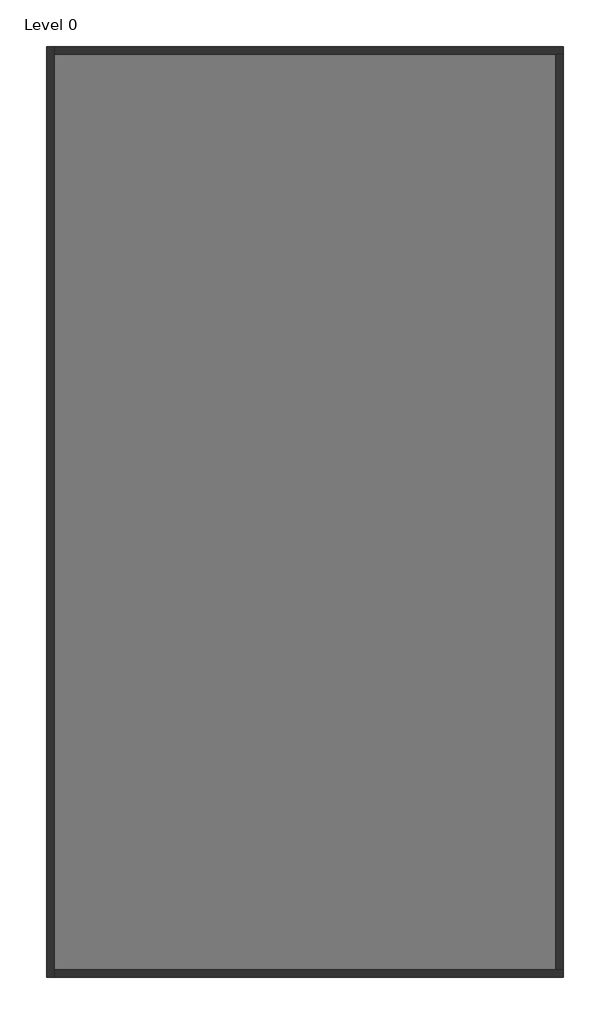
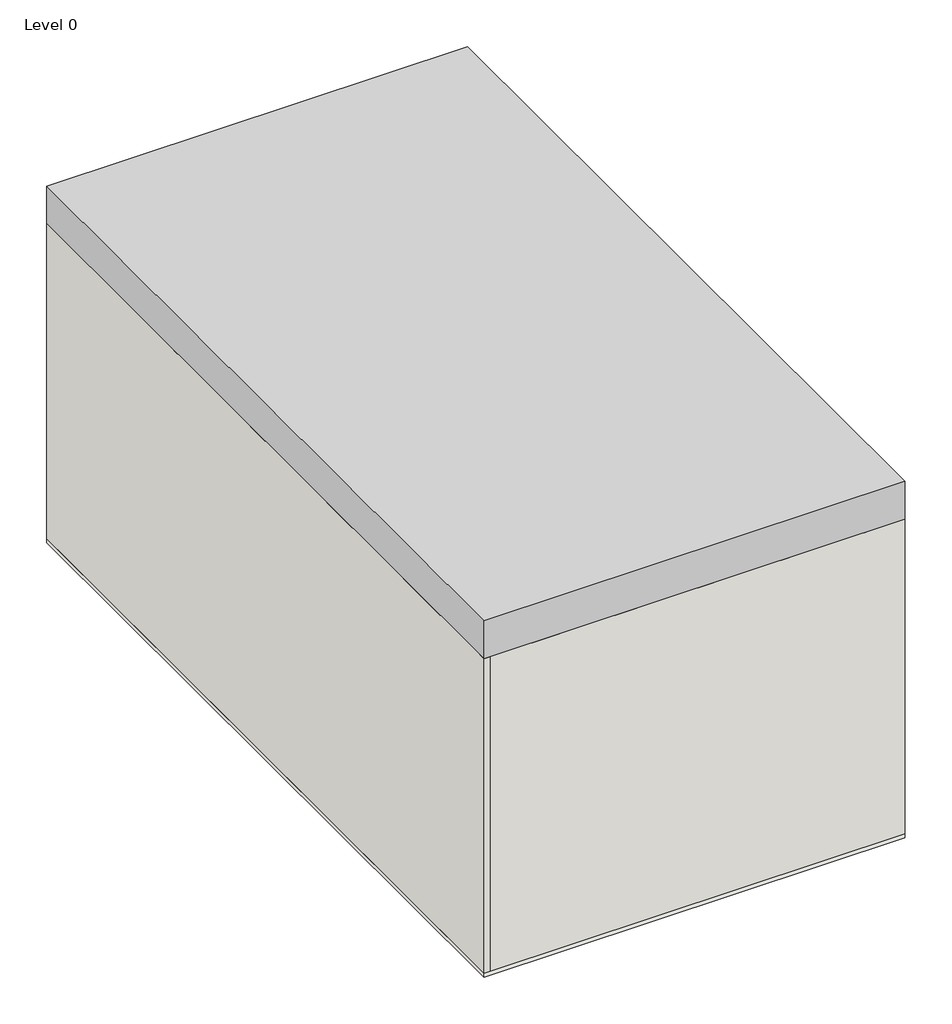
# One storey: 4 walls, 1 proxy, 1 slab.
"""IFC4 building model written with IfcOpenShell, lengths in millimetres."""

from ifc_helpers import new_model, si_unit, frame, origin, origin_with_axes, place, context, project, spatial, polyline, outline, extrude, faceted_brep, element, save

model = new_model("IFC4")

# Units and contexts
model_context = context("Model", 3, world=origin())
ifc_project = project(units=[si_unit("LENGTHUNIT", "METRE", prefix="MILLI")], contexts=[model_context])

# Site, building, storey
site = spatial("IfcSite", under=ifc_project)
building = spatial("IfcBuilding", under=site)
storey = spatial("IfcBuildingStorey", under=building, Name="Level 0", Elevation=100.0)

# Proxy
placement = place(None, origin())
element("IfcBuildingElementProxy", 1, Name="LowUrbanDensityBuilding : LowUrbanDensityBuilding", ObjectType="LowUrbanDensityBuilding : LowUrbanDensityBuilding", at=placement, inside=storey, context=model_context, shape_type="SweptSolid", body=[
    extrude(outline(polyline([(7325.2659446, 3676.2074539), (7325.2659446, -14323.7925461), (-2674.7340554, -14323.7925461), (-2674.7340554, 3676.2074539), (7325.2659446, 3676.2074539)])), origin_with_axes(), (0.0, 0.0, 1.0), 8949.8),
])

# Slab
element("IfcSlab", 2, ObjectType="Floor-Concrete_100Con", at=placement, inside=storey, context=model_context, shape_type="SweptSolid", body=[
    extrude(outline(polyline([(7325.2659446, 3676.2074539), (7325.2659446, -14323.7925461), (-2674.7340554, -14323.7925461), (-2674.7340554, 3676.2074539), (7325.2659446, 3676.2074539)])), origin_with_axes(), (0.0, 0.0, 1.0), 100.0),
])

# Walls
element("IfcWall", 3, ObjectType="Wall-Ext_25Rdr-100Blk-19P", at=placement, inside=storey, context=model_context, shape_type="Brep", body=[
    faceted_brep([(-2674.7340554, 3676.2074539, 100.0), (-2674.7340554, -14323.7925461, 100.0), (-2674.7340554, -14323.7925461, 8000.0), (-2674.7340554, 3676.2074539, 8000.0), (-2530.4340554, 3676.2074539, 100.0), (-2530.4340554, 3676.2074539, 8000.0), (-2530.4340554, 3531.9074539, 8000.0), (-2530.4340554, -14179.4925461, 8000.0), (-2530.4340554, -14323.7925461, 8000.0), (-2530.4340554, -14323.7925461, 100.0), (-2530.4340554, -14179.4925461, 100.0), (-2530.4340554, 3531.9074539, 100.0)], [[[0, 1, 2, 3]], [[4, 5, 6, 7, 8, 9, 10, 11]], [[1, 0, 4, 11, 10, 9]], [[3, 2, 8, 7, 6, 5]], [[2, 1, 9, 8]], [[0, 3, 5, 4]]]),
])
element("IfcWall", 4, ObjectType="Wall-Ext_25Rdr-100Blk-19P", at=placement, inside=storey, context=model_context, shape_type="Brep", body=[
    faceted_brep([(-2530.4340554, -14323.7925461, 100.0), (7325.2659446, -14323.7925461, 100.0), (7325.2659446, -14323.7925461, 8000.0), (-2530.4340554, -14323.7925461, 8000.0), (-2530.4340554, -14179.4925461, 100.0), (-2530.4340554, -14179.4925461, 8000.0), (7180.9659446, -14179.4925461, 8000.0), (7325.2659446, -14179.4925461, 8000.0), (7325.2659446, -14179.4925461, 100.0), (7180.9659446, -14179.4925461, 100.0)], [[[0, 1, 2, 3]], [[4, 5, 6, 7, 8, 9]], [[1, 0, 4, 9, 8]], [[3, 2, 7, 6, 5]], [[0, 3, 5, 4]], [[2, 1, 8, 7]]]),
])
element("IfcWall", 5, ObjectType="Wall-Ext_25Rdr-100Blk-19P", at=placement, inside=storey, context=model_context, shape_type="Brep", body=[
    faceted_brep([(7325.2659446, 3676.2074539, 100.0), (-2530.4340554, 3676.2074539, 100.0), (-2530.4340554, 3676.2074539, 8000.0), (7325.2659446, 3676.2074539, 8000.0), (7325.2659446, 3531.9074539, 100.0), (7325.2659446, 3531.9074539, 8000.0), (7180.9659446, 3531.9074539, 8000.0), (-2530.4340554, 3531.9074539, 8000.0), (-2530.4340554, 3531.9074539, 100.0), (7180.9659446, 3531.9074539, 100.0)], [[[0, 1, 2, 3]], [[4, 5, 6, 7, 8, 9]], [[1, 0, 4, 9, 8]], [[3, 2, 7, 6, 5]], [[2, 1, 8, 7]], [[0, 3, 5, 4]]]),
])
element("IfcWall", 6, ObjectType="Wall-Ext_25Rdr-100Blk-19P", at=placement, inside=storey, context=model_context, shape_type="SweptSolid", body=[
    extrude(outline(polyline([(7325.2659446, 3531.9074539), (7325.2659446, -14179.4925461), (7180.9659446, -14179.4925461), (7180.9659446, 3531.9074539), (7325.2659446, 3531.9074539)])), frame((0.0, 0.0, 100.0), z_axis=(0.0, 0.0, 1.0), x_axis=(1.0, 0.0, 0.0)), (0.0, 0.0, 1.0), 7900.0),
])

save(model, "model.ifc")

# Revit data of these elements
# Project information
#   Project Issue Date = "Issue Date"
#   Project Status = "Project Status"
#   Client Name = "Owner"
#   Project Address = "Enter address here"
#   Project Name = "Project Name"
#   Project Number = "Project Number"
# Type "Floor-Concrete_100Con"
#   Keynote = "E60/130"
#   Function = 0
#   Layers, outside or top first: 100 mm "Concrete" (function 1)
# Type "Wall-Ext_25Rdr-100Blk-19P"
#   Keynote = "F10"
#   Layers, outside or top first: 25.3 mm "Render, Beige, Smooth" (function 5); 100 mm "Concrete Masonry Units _Low Density" (function 1); 19 mm "Plaster" (function 5)
# Element 1 (IfcBuildingElementProxy, "LowUrbanDensityBuilding : LowUrbanDensityBuilding")
#   Phase Created = New Construction
#   Materials on its faces: "Default Form"
# Element 2 (IfcSlab, "Floor-Concrete_100Con")
#   Height Offset From Level = 0 mm
#   Phase Created = New Construction
#   Materials on its faces: "Concrete"
# Element 3 (IfcWall, "Wall-Ext_25Rdr-100Blk-19P")
#   Top Offset = 0 mm
#   Base Offset = 0 mm
#   wall height = 7900 mm
#   Phase Created = New Construction
#   Base Constraint = Level 0
#   Top Constraint = Level 2
#   Materials on its faces: "Render, Beige, Smooth", "Default Wall", "Plaster"
# Elements 4, 5, 6 (IfcWall, "Wall-Ext_25Rdr-100Blk-19P")
#   Top Offset = 0 mm
#   Base Offset = 0 mm
#   wall height = 7900 mm
#   Phase Created = New Construction
#   Base Constraint = Level 0
#   Top Constraint = Level 2
#   Materials on its faces: "Default Wall", "Render, Beige, Smooth", "Plaster"
# Materials
#   "Concrete": class "Concrete", colour RGB 120 120 120, transparency 0, Description = "Portland Cement Concrete", Cost = 0
#   "Render, Beige, Smooth": class "Generic", colour RGB 213 198 180, transparency 0, Description = "physical material", Cost = 0
#   "Concrete Masonry Units _Low Density": class "Masonry", colour RGB 181 181 181, transparency 0, Description = "Concrete masonry units", Cost = 0
#   "Plaster": class "Generic", colour RGB 249 249 249, transparency 0, Description = "Plaster", Cost = 0
#   "Default Form": class "Generic", colour RGB 185 189 196, transparency 0.5, Cost = 0
#   "Default Wall": class "Miscellaneous", colour RGB 128 128 128, transparency 0, Comments = "Rendering appearance not upgraded Rendering appearance not upgraded ", Cost = 0
